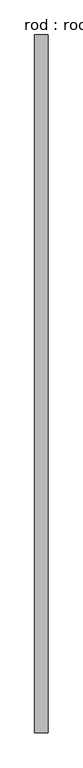
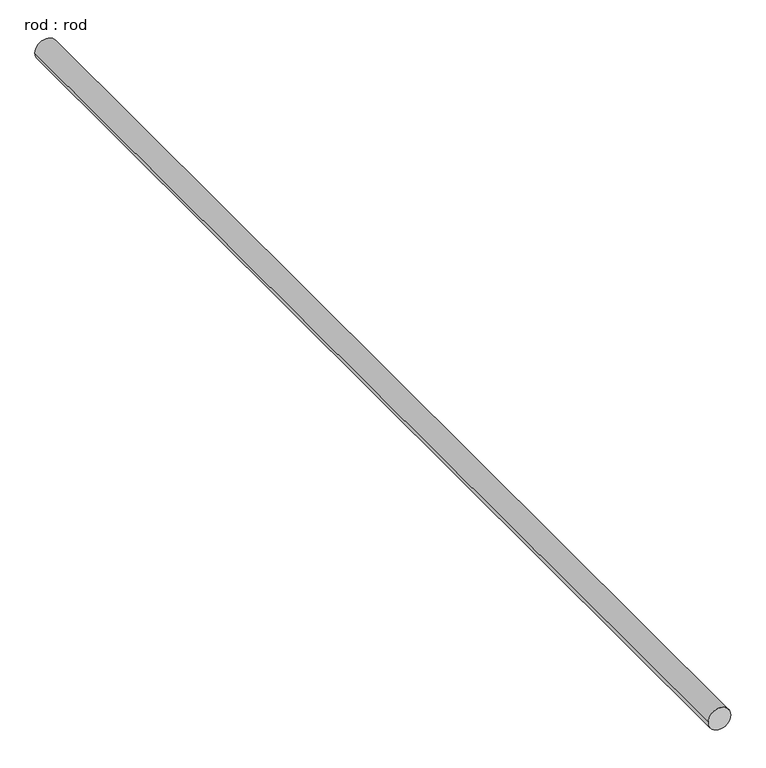
"""IFC4 building model written with IfcOpenShell, lengths in millimetres: proxy geometry, rod : rod."""

from ifc_helpers import new_model, si_unit, point, frame, frame_2d, origin, place, context, project, spatial, circle_curve, trimmed, segment, composite_curve, outline, extrude, source, transform, mapped, element, save


def rod_rod_5089427b(model_context):
    return source(origin(), model_context, "Body", "SweptSolid", [
        extrude(outline(composite_curve([segment(trimmed(circle_curve(frame_2d((0.0108462, 0.0)), 200.0), [point((0.0108462, 200.0))], [point((0.0108462, -200.0))], False, "CARTESIAN"), True, "CONTINUOUS"), segment(trimmed(circle_curve(frame_2d((0.0108462, 0.0)), 200.0), [point((0.0108462, -200.0))], [point((0.0108462, 200.0))], False, "CARTESIAN"), True, "CONTINUOUS")], self_intersect=False)), frame((0.0, -6214.611875, 0.0), z_axis=(0.0, 1.0, 0.0), x_axis=(0.0, 0.0, 1.0)), (0.0, 0.0, 1.0), 20614.6809808),
    ])


if __name__ == "__main__":
    model = new_model("IFC4")
    model_context = context("Model", 3, world=origin())
    ifc_project = project(units=[si_unit("LENGTHUNIT", "METRE", prefix="MILLI")], contexts=[model_context])
    site = spatial("IfcSite", under=ifc_project)
    building = spatial("IfcBuilding", under=site)
    placement = place(None, origin())
    rod_rod_shape = rod_rod_5089427b(model_context)
    element("IfcBuildingElementProxy", 1, Name="rod : rod", ObjectType="rod : rod", at=placement, inside=building, context=model_context, shape_type="MappedRepresentation", body=[
        mapped(rod_rod_shape, transform((0.0, 0.0, 0.0), x_axis=(1.0, 0.0, 0.0), y_axis=(0.0, 1.0, 0.0), z_axis=(0.0, 0.0, 1.0))),
    ])
    save(model, "model.ifc")

# Revit data of these elements
# Type "rod : rod"
#   Default Elevation = 0
